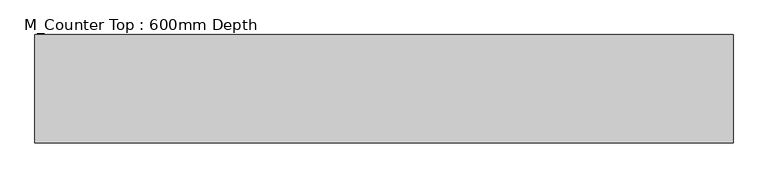
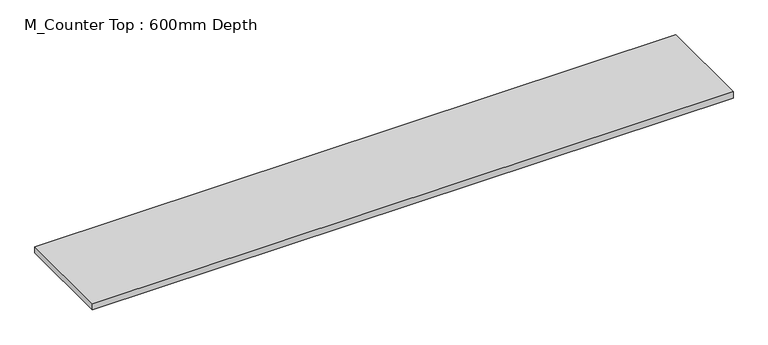
"""IFC4 building model written with IfcOpenShell, lengths in millimetres: furniture geometry, M_Counter Top : 600mm Depth."""

import ifcopenshell
import ifcopenshell.guid

model = None  # the IFC model being written
_history = None  # IfcOwnerHistory: only IFC2X3 demands one
_inside = {}  # id of a spatial element -> (the spatial element, [elements in it])
_under = {}  # id of a project, library or spatial element -> (it, [spatial elements below it])
_declared = {}  # id of a project -> (the project, [libraries it declares])
_typed = {}  # id of a type object -> (the type object, [elements of that type])
_made_of = {}  # id of a material, layer set ... -> (it, [elements and type objects made of it])


def new_model(schema):
    """Start an empty IFC model of exactly this schema.

    Asked for "IFC4X3", IfcOpenShell would pick the latest addendum, in which some entities
    have other attributes; the version numbers below select the first issue.
    IFC2X3 requires an IfcOwnerHistory on every rooted entity: one is made here for all.
    """
    global model, _history
    if schema == "IFC4X3":
        model = ifcopenshell.file(schema_version=(4, 3, 0, 0))
    else:
        model = ifcopenshell.file(schema=schema)
    _inside.clear()
    _under.clear()
    _declared.clear()
    _typed.clear()
    _made_of.clear()
    _history = None
    if model.schema == "IFC2X3":
        org = make("IfcOrganization", Name="unknown")
        user = make(
            "IfcPersonAndOrganization",
            ThePerson=make("IfcPerson", FamilyName="unknown"),
            TheOrganization=org,
        )
        app = make(
            "IfcApplication",
            ApplicationDeveloper=org,
            Version="unknown",
            ApplicationFullName="unknown",
            ApplicationIdentifier="unknown",
        )
        _history = make(
            "IfcOwnerHistory",
            OwningUser=user,
            OwningApplication=app,
            ChangeAction="ADDED",
            CreationDate=0,
        )
    return model


def make(cls, **values):
    """One entity of the class cls with the attributes given. An attribute that is None is left unset."""
    return model.create_entity(
        cls, **{name: value for name, value in values.items() if value is not None}
    )


def rooted(cls, **values):
    """An entity with a GlobalId (a new one), such as an element, a storey or a relation."""
    return make(cls, GlobalId=ifcopenshell.guid.new(), OwnerHistory=_history, **values)


def si_unit(unit_type, name, prefix=None):
    """IfcSIUnit, for example si_unit("LENGTHUNIT", "METRE", prefix="MILLI")."""
    return make("IfcSIUnit", UnitType=unit_type, Prefix=prefix, Name=name)


def assignment(units):
    """IfcUnitAssignment: the units of a project."""
    return None if units is None else make("IfcUnitAssignment", Units=units)


def point(xyz):
    """IfcCartesianPoint."""
    return None if xyz is None else make("IfcCartesianPoint", Coordinates=xyz)


def direction(xyz):
    """IfcDirection."""
    return None if xyz is None else make("IfcDirection", DirectionRatios=xyz)


def frame(location, z_axis=None, x_axis=None):
    """IfcAxis2Placement3D, a coordinate frame: its origin and axes. An axis left out is left unset."""
    return make(
        "IfcAxis2Placement3D",
        Location=point(location),
        Axis=direction(z_axis),
        RefDirection=direction(x_axis),
    )


def origin():
    """The frame at (0, 0, 0) with its axes left unset."""
    return frame((0.0, 0.0, 0.0))


def place(relative_to, where):
    """IfcLocalPlacement: puts the frame where relative to a parent placement (None: the world)."""
    return make(
        "IfcLocalPlacement", PlacementRelTo=relative_to, RelativePlacement=where
    )


def context(
    kind, dimensions, precision=None, world=None, true_north=None, identifier=None
):
    """IfcGeometricRepresentationContext, for example the 3D "Model" context."""
    return make(
        "IfcGeometricRepresentationContext",
        ContextIdentifier=identifier,
        ContextType=kind,
        CoordinateSpaceDimension=dimensions,
        Precision=precision,
        WorldCoordinateSystem=world,
        TrueNorth=true_north,
    )


def project(units=None, contexts=None):
    """IfcProject with its units and contexts."""
    return rooted(
        "IfcProject",
        Name="project",
        RepresentationContexts=contexts,
        UnitsInContext=assignment(units),
    )


def spatial(cls, under=None, at=None, **own):
    """A site, building, storey or space (cls), placed at a placement, below another one or the project."""
    s = rooted(cls, ObjectPlacement=at, **own)
    if under is not None:
        _under.setdefault(under.id(), (under, []))[1].append(s)
    return s


def polyline(points):
    """IfcPolyline through the points."""
    return make("IfcPolyline", Points=[point(p) for p in points])


def outline(outer, holes=None, kind="AREA"):
    """IfcArbitraryClosedProfileDef: a profile drawn as a closed curve; with holes, ...WithVoids."""
    if holes is None:
        return make("IfcArbitraryClosedProfileDef", ProfileType=kind, OuterCurve=outer)
    return make(
        "IfcArbitraryProfileDefWithVoids",
        ProfileType=kind,
        OuterCurve=outer,
        InnerCurves=holes,
    )


def extrude(swept, where, along, depth):
    """IfcExtrudedAreaSolid: the profile swept, set in the frame where, extruded along a direction by depth."""
    return make(
        "IfcExtrudedAreaSolid",
        SweptArea=swept,
        Position=where,
        ExtrudedDirection=direction(along),
        Depth=depth,
    )


def shape(context_of_items, identifier, shape_type, items):
    """IfcShapeRepresentation: the items that make up one representation, for example the "Body"."""
    return make(
        "IfcShapeRepresentation",
        ContextOfItems=context_of_items,
        RepresentationIdentifier=identifier,
        RepresentationType=shape_type,
        Items=items,
    )


def source(mapping_origin, context_of_items, identifier, shape_type, items):
    """IfcRepresentationMap: a shape defined once, which mapped items show again and again."""
    return make(
        "IfcRepresentationMap",
        MappingOrigin=mapping_origin,
        MappedRepresentation=shape(context_of_items, identifier, shape_type, items),
    )


def transform(
    local_origin,
    x_axis=None,
    y_axis=None,
    z_axis=None,
    scale=None,
    scale2=None,
    scale3=None,
    uniform=True,
):
    """IfcCartesianTransformationOperator3D, or its non-uniform kind. x_axis, y_axis, z_axis: its Axis1, 2, 3."""
    if uniform:
        return make(
            "IfcCartesianTransformationOperator3D",
            Axis1=direction(x_axis),
            Axis2=direction(y_axis),
            LocalOrigin=point(local_origin),
            Scale=scale,
            Axis3=direction(z_axis),
        )
    return make(
        "IfcCartesianTransformationOperator3DnonUniform",
        Axis1=direction(x_axis),
        Axis2=direction(y_axis),
        LocalOrigin=point(local_origin),
        Scale=scale,
        Axis3=direction(z_axis),
        Scale2=scale2,
        Scale3=scale3,
    )


def mapped(mapping_source, mapping_target):
    """IfcMappedItem: shows the shape of a source again, moved by a transform."""
    return make(
        "IfcMappedItem", MappingSource=mapping_source, MappingTarget=mapping_target
    )


def made_of(thing, what):
    """Note that an element or type object is made of a material, layer set ...; save() writes the relation."""
    if what is not None:
        _made_of.setdefault(what.id(), (what, []))[1].append(thing)
    return thing


def element(
    cls,
    number,
    at=None,
    inside=None,
    cuts=None,
    type_object=None,
    material=None,
    context=None,
    identifier="Body",
    shape_type=None,
    held_by="IfcProductDefinitionShape",
    body=None,
    shapes=None,
    **own,
):
    """One element of the class cls, such as IfcWall. Its Tag is "e" and its number.

    at: its placement. inside: the storey or other place that contains it. cuts: it is an
    opening in that element (IfcRelVoidsElement). A single representation is given by context,
    identifier, shape_type and body (its items); several are given by shapes. held_by: the class
    of the entity that holds the representations. save() writes the other relations.
    """
    e = rooted(cls, Tag="e%d" % number, ObjectPlacement=at, **own)
    if body is not None:
        shapes = [shape(context, identifier, shape_type, body)]
    if shapes is not None:
        e.Representation = make(held_by, Representations=shapes)
    if inside is not None:
        _inside.setdefault(inside.id(), (inside, []))[1].append(e)
    if cuts is not None:
        rooted(
            "IfcRelVoidsElement", RelatingBuildingElement=cuts, RelatedOpeningElement=e
        )
    if type_object is not None:
        _typed.setdefault(type_object.id(), (type_object, []))[1].append(e)
    return made_of(e, material)


def aggregate(whole, parts):
    """IfcRelAggregates: a whole, such as a stair, and the parts it consists of."""
    return rooted("IfcRelAggregates", RelatingObject=whole, RelatedObjects=parts)


def save(model, path):
    """Write the relations noted so far, then the file.

    IfcRelAggregates (storeys below a building ...), IfcRelContainedInSpatialStructure (elements
    in a storey), IfcRelDefinesByType, IfcRelAssociatesMaterial and IfcRelDeclares: one each for
    every whole, place, type object, material and project.
    """
    for whole, parts in _under.values():
        aggregate(whole, parts)
    for where, things in _inside.values():
        rooted(
            "IfcRelContainedInSpatialStructure",
            RelatedElements=things,
            RelatingStructure=where,
        )
    for kind, things in _typed.values():
        rooted("IfcRelDefinesByType", RelatedObjects=things, RelatingType=kind)
    for what, things in _made_of.values():
        rooted("IfcRelAssociatesMaterial", RelatedObjects=things, RelatingMaterial=what)
    for by, libraries in _declared.values():
        rooted("IfcRelDeclares", RelatingContext=by, RelatedDefinitions=libraries)
    model.write(path)


def m_counter_top_600mm_depth_a21ada81(model_context):
    return source(origin(), model_context, "Body", "SweptSolid", [
        extrude(outline(polyline([(2823.5377049, 0.0), (2823.5377049, -625.0), (-1200.4622951, -625.0), (-1200.4622951, 0.0), (2823.5377049, 0.0)])), frame((0.0, 0.0, 860.0), z_axis=(0.0, 0.0, 1.0), x_axis=(1.0, 0.0, 0.0)), (0.0, 0.0, 1.0), 40.0),
    ])


if __name__ == "__main__":
    model = new_model("IFC4")
    model_context = context("Model", 3, world=origin())
    ifc_project = project(units=[si_unit("LENGTHUNIT", "METRE", prefix="MILLI")], contexts=[model_context])
    site = spatial("IfcSite", under=ifc_project)
    building = spatial("IfcBuilding", under=site)
    placement = place(None, origin())
    m_counter_top_600mm_depth_shape = m_counter_top_600mm_depth_a21ada81(model_context)
    element("IfcFurniture", 1, ObjectType="M_Counter Top : 600mm Depth", at=placement, inside=building, context=model_context, shape_type="MappedRepresentation", body=[
        mapped(m_counter_top_600mm_depth_shape, transform((0.0, 0.0, 0.0), x_axis=(1.0, 0.0, 0.0), y_axis=(0.0, 1.0, 0.0), z_axis=(0.0, 0.0, 1.0))),
    ])
    save(model, "model.ifc")

# Revit data of these elements
# Type "M_Counter Top : 600mm Depth"
#   AccessibilityPerformance = "AccessibilityPerformance"
#   CodePerformance = "CodePerformance"
#   Area = "Area"
#   Color = "Color"
#   Constituents = "Constituents"
#   Features = "Features"
#   Finish = "Finish"
#   Grade = "Grade"
#   Material = "Material"
#   ModelReference = "ModelReference"
#   NominalHeight = "NominalHeight"
#   NominalLength = "NominalLength"
#   NominalWidth = "NominalWidth"
#   ProductionYear = "ProductionYear"
#   Reference = "Reference"
#   Shape = "Shape"
#   Size = "Size"
#   SustainabilityPerformance = "SustainabilityPerformance"
#   WarrantyDescription = "WarrantyDescription"
#   WarrantyDurationLabor = "WarrantyDurationLabor"
#   WarrantyDurationParts = "WarrantyDurationParts"
#   WarrantyGuarantorLabor = "WarrantyGuarantorLabor"
#   WarrantyGuarantorParts = "WarrantyGuarantorParts"
#   ExpectedLife = "ExpectedLife"
#   ReplacementCost = "ReplacementCost"
#   AssetAccountingType = "FIXED"
#   ModelLabel = "ModelLabel"
#   Manufacturer = "Manufacturer"
#   Finish = "Finish"
#   Construction Type = "Construction Type"
#   Counter Thickness = 0.040 m
#   Depth = 0.625 m
#   Height = 0.900 m
#   Length [instance default] = 2.500 m
#   Backsplash Visibility [instance default] = yes
#   Counter Top Material = none
#   Assembly Code = ""
# Element 1 (IfcFurniture, "M_Counter Top : 600mm Depth")
#   Length = 4.024 m
#   Backsplash Visibility = no
#   Materials on its faces: "Counter Top"
# Materials
#   "Counter Top": class "Wood", colour RGB 226 177 128, transparency 0
